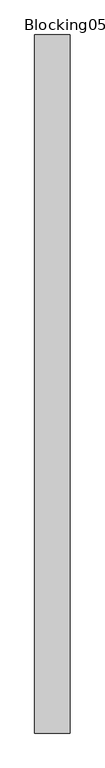
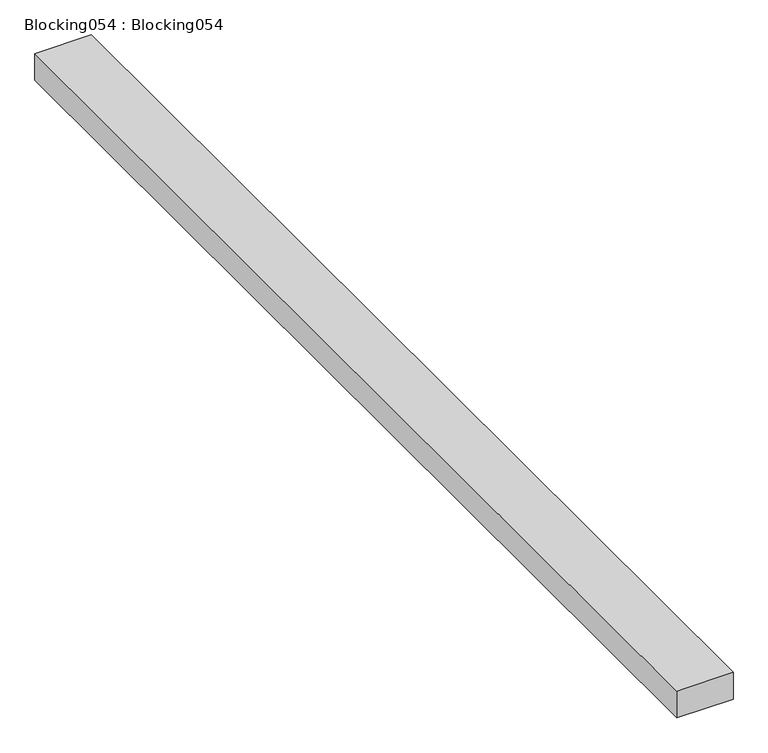
"""IFC4 building model written with IfcOpenShell, lengths in millimetres: proxy geometry, Blocking054 : Blocking054."""

from ifc_helpers import new_model, si_unit, frame, origin, place, context, project, spatial, polyline, outline, extrude, source, transform, mapped, element, save


def blocking054_blocking054_5621276c(model_context):
    return source(origin(), model_context, "Body", "SweptSolid", [
        extrude(outline(polyline([(-9787.3237014, 7982.1531721), (-9888.9237014, 7982.1531721), (-9888.9237014, 9982.1531721), (-9787.3237014, 9982.1531721), (-9787.3237014, 7982.1531721)])), frame((0.0, 0.0, 40106.3460083), z_axis=(0.0, 0.0, 1.0), x_axis=(1.0, 0.0, 0.0)), (0.0, 0.0, 1.0), 50.8),
    ])


if __name__ == "__main__":
    model = new_model("IFC4")
    model_context = context("Model", 3, world=origin())
    ifc_project = project(units=[si_unit("LENGTHUNIT", "METRE", prefix="MILLI")], contexts=[model_context])
    site = spatial("IfcSite", under=ifc_project)
    building = spatial("IfcBuilding", under=site)
    placement = place(None, origin())
    blocking054_blocking054_shape = blocking054_blocking054_5621276c(model_context)
    element("IfcBuildingElementProxy", 1, Name="Blocking054 : Blocking054", ObjectType="Blocking054 : Blocking054", at=placement, inside=building, context=model_context, shape_type="MappedRepresentation", body=[
        mapped(blocking054_blocking054_shape, transform((0.0, 0.0, 0.0), x_axis=(1.0, 0.0, 0.0), y_axis=(0.0, 1.0, 0.0), z_axis=(0.0, 0.0, 1.0))),
    ])
    save(model, "model.ifc")

# Revit data of these elements
# Type "Blocking054 : Blocking054"
#   NameOverride = "Blocking054"
# Element 1 (IfcBuildingElementProxy, "Blocking054 : Blocking054")
#   Materials on its faces: "WOOD BLOCKING AS REQUIRED"
# Materials
#   "WOOD BLOCKING AS REQUIRED": class "Unassigned", colour RGB 166 124 85, transparency 0, Cost = 0
